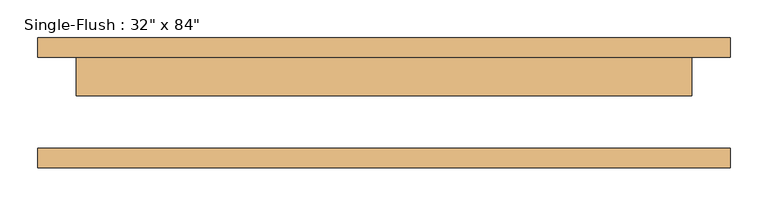
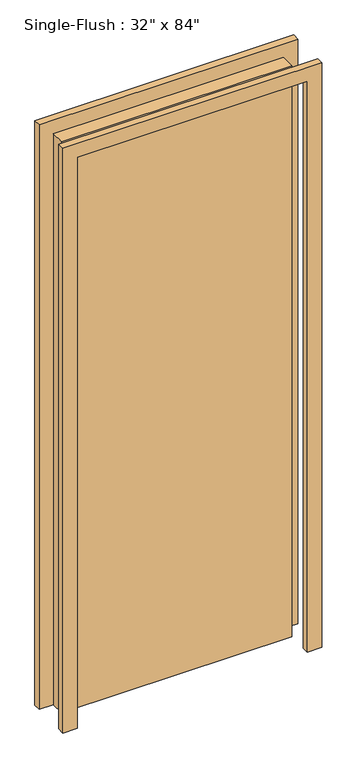
"""IFC4 building model written with IfcOpenShell, lengths in millimetres: door geometry."""

from ifc_helpers import new_model, si_unit, frame, origin, origin_with_axes, place, context, project, spatial, polyline, outline, extrude, source, transform, mapped, element, save


def door_2cba8012(model_context):
    return source(origin(), model_context, "Body", "SweptSolid", [
        extrude(outline(polyline([(2184.4, -457.2), (0.0, -457.2), (0.0, -406.4), (2133.6, -406.4), (2133.6, 406.4), (0.0, 406.4), (0.0, 457.2), (2184.4, 457.2), (2184.4, -457.2)])), frame((0.0, 60.325, 0.0), z_axis=(0.0, 1.0, 0.0), x_axis=(0.0, 0.0, 1.0)), (0.0, 0.0, 1.0), 25.4),
        extrude(outline(polyline([(2184.4, 457.2), (2184.4, -457.2), (0.0, -457.2), (0.0, -406.4), (2133.6, -406.4), (2133.6, 406.4), (0.0, 406.4), (0.0, 457.2), (2184.4, 457.2)])), frame((0.0, -85.725, 0.0), z_axis=(0.0, 1.0, 0.0), x_axis=(0.0, 0.0, 1.0)), (0.0, 0.0, 1.0), 25.4),
        extrude(outline(polyline([(406.4, 9.525), (-406.4, 9.525), (-406.4, 60.325), (406.4, 60.325), (406.4, 9.525)])), origin_with_axes(), (0.0, 0.0, 1.0), 2133.6),
    ])


if __name__ == "__main__":
    model = new_model("IFC4")
    model_context = context("Model", 3, world=origin())
    ifc_project = project(units=[si_unit("LENGTHUNIT", "METRE", prefix="MILLI")], contexts=[model_context])
    site = spatial("IfcSite", under=ifc_project)
    building = spatial("IfcBuilding", under=site)
    placement = place(None, origin())
    door_shape = door_2cba8012(model_context)
    element("IfcDoor", 1, ObjectType="Single-Flush : 32\" x 84\"", at=placement, inside=building, context=model_context, shape_type="MappedRepresentation", body=[
        mapped(door_shape, transform((0.0, 0.0, 0.0), x_axis=(1.0, 0.0, 0.0), y_axis=(0.0, 1.0, 0.0), z_axis=(0.0, 0.0, 1.0))),
    ])
    save(model, "model.ifc")

# Revit data of these elements
# Type "Single-Flush : 32\" x 84\""
#   Type Mark = "10"
#   Construction Type Id = "MDOOR"
#   Assembly Code = "C1020"
#   Analytic Construction = "Metal"
#   Thickness = 0' - 2"
#   Heat Transfer Coefficient (U) = 3.7021 W/(m²·K)
#   Height = 7' - 0"
#   Trim Projection Ext = 0' - 1"
#   Trim Projection Int = 0' - 1"
#   Trim Width = 0' - 2"
#   Width = 2' - 8"
#   Door Material = Door - Panel
#   Frame Material = Door - Frame
#   Visual Light Transmittance = 0
#   Solar Heat Gain Coefficient = 0
#   Function = (empty or 0)
#   Wall Closure = (empty or 0)
# Element 1 (IfcDoor, "Single-Flush : 32\" x 84\"")
#   Materials on its faces: "Door - Frame", "Door - Panel"
# Materials
#   "Door - Panel": class "Wood", colour RGB 212 179 113, transparency 0, Cost = 0
#   "Door - Frame": class "Miscellaneous", colour RGB 65 65 65, transparency 0, Cost = 0
